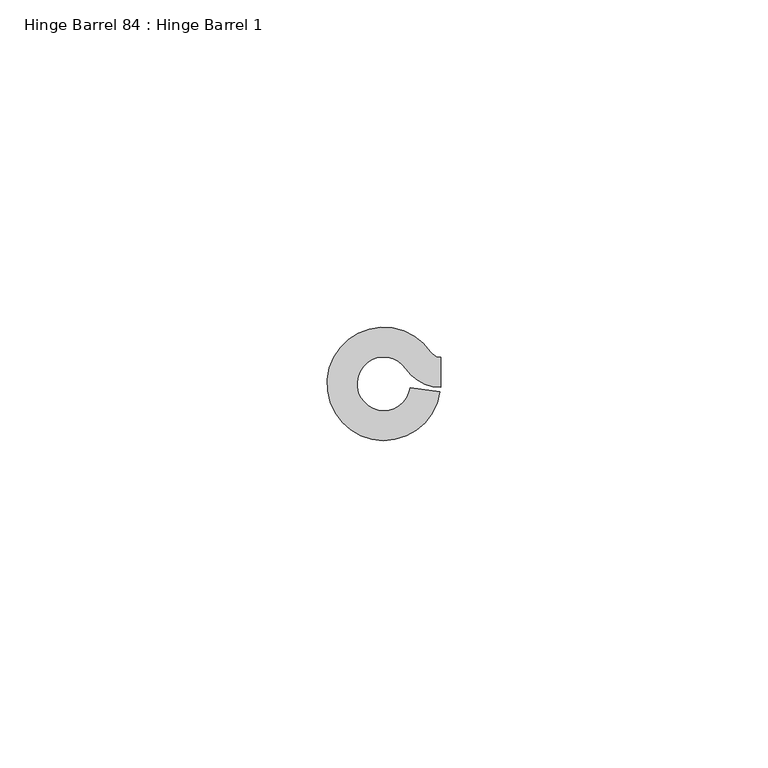
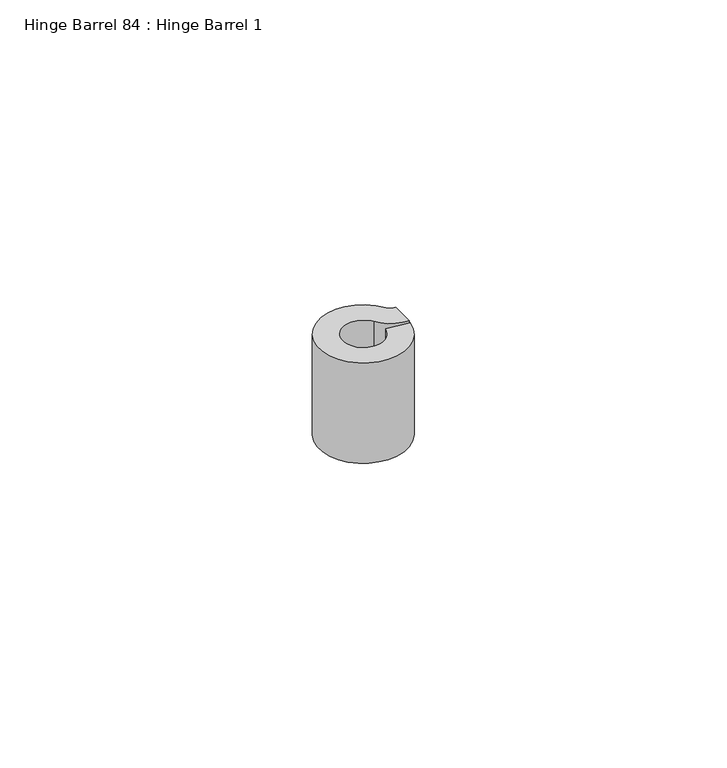
"""IFC4 building model written with IfcOpenShell, lengths in millimetres: proxy geometry, Hinge Barrel 84 : Hinge Barrel 1."""

from ifc_helpers import new_model, si_unit, point, frame, frame_2d, origin, place, context, project, spatial, polyline, circle_curve, trimmed, segment, composite_curve, outline, extrude, source, transform, mapped, element, save


def hinge_barrel_84_hinge_barrel_1_babfa127(model_context):
    return source(origin(), model_context, "Body", "SweptSolid", [
        extrude(outline(composite_curve([segment(trimmed(circle_curve(frame_2d((587319.1320739, -531776.6049841)), 4.0894), [point((587322.5194669, -531774.3139665))], [point((587323.1821338, -531777.1708529))], True, "CARTESIAN"), True, "CONTINUOUS"), segment(polyline([(587323.1821338, -531777.1708529), (587327.7022899, -531777.8024028)]), True, "CONTINUOUS"), segment(trimmed(circle_curve(frame_2d((587319.1320739, -531776.6049841)), 8.6534625), [point((587327.7022899, -531777.8024028))], [point((587326.3000393, -531771.7570273))], False, "CARTESIAN"), True, "CONTINUOUS"), segment(trimmed(circle_curve(frame_2d((587327.8245257, -531770.7259615)), 1.8404226), [point((587326.3000393, -531771.7570273))], [point((587327.8245257, -531772.5663841))], True, "CARTESIAN"), True, "CONTINUOUS"), segment(polyline([(587327.8245257, -531772.5663841), (587327.8245257, -531777.1304466)]), True, "CONTINUOUS"), segment(trimmed(circle_curve(frame_2d((587327.8245257, -531770.7259615)), 6.4044851), [point((587327.8245257, -531777.1304466))], [point((587322.5194669, -531774.3139665))], False, "CARTESIAN"), True, "CONTINUOUS")], self_intersect=False)), frame((0.0, 0.0, 2063.75), z_axis=(0.0, 0.0, 1.0), x_axis=(1.0, 0.0, 0.0)), (0.0, 0.0, 1.0), 20.8359375),
    ])


if __name__ == "__main__":
    model = new_model("IFC4")
    model_context = context("Model", 3, world=origin())
    ifc_project = project(units=[si_unit("LENGTHUNIT", "METRE", prefix="MILLI")], contexts=[model_context])
    site = spatial("IfcSite", under=ifc_project)
    building = spatial("IfcBuilding", under=site)
    placement = place(None, origin())
    hinge_barrel_84_hinge_barrel_1_shape = hinge_barrel_84_hinge_barrel_1_babfa127(model_context)
    element("IfcBuildingElementProxy", 1, Name="Hinge Barrel 84 : Hinge Barrel 1", ObjectType="Hinge Barrel 84 : Hinge Barrel 1", at=placement, inside=building, context=model_context, shape_type="MappedRepresentation", body=[
        mapped(hinge_barrel_84_hinge_barrel_1_shape, transform((0.0, 0.0, 0.0), x_axis=(1.0, 0.0, 0.0), y_axis=(0.0, 1.0, 0.0), z_axis=(0.0, 0.0, 1.0))),
    ])
    save(model, "model.ifc")

# Revit data of these elements
# Element 1 (IfcBuildingElementProxy, "Hinge Barrel 84 : Hinge Barrel 1")
#   Materials on its faces: "6\"X6\" WELD-ON STL BUTT HINGE"
# Materials
#   "6\"X6\" WELD-ON STL BUTT HINGE": class "Metal", colour RGB 189 187 185, transparency 0, Description = "Carbon steel", Cost = 0
